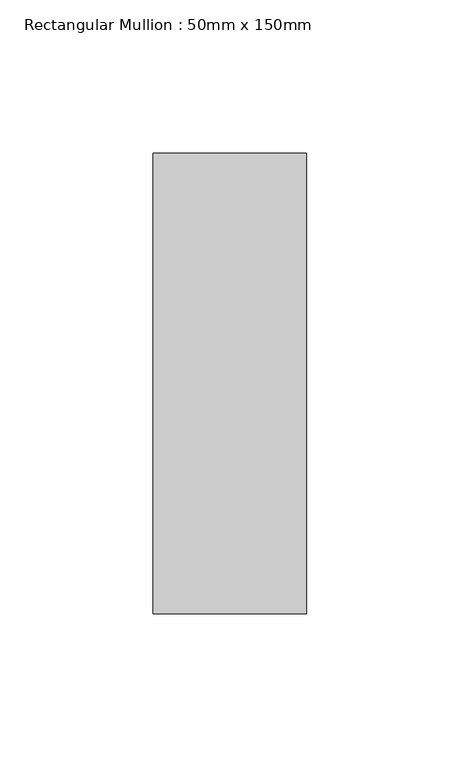
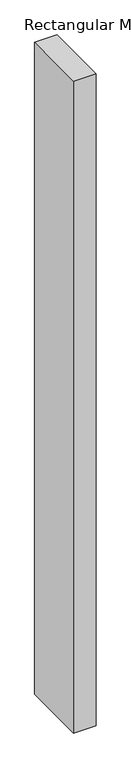
"""IFC4 building model written with IfcOpenShell, lengths in millimetres: member geometry, Rectangular Mullion : 50mm x 150mm."""

from ifc_helpers import new_model, si_unit, frame, origin, place, context, project, spatial, polyline, outline, extrude, source, transform, mapped, element, save


def rectangular_mullion_50mm_x_150mm_95afd124(model_context):
    return source(origin(), model_context, "Body", "SweptSolid", [
        extrude(outline(polyline([(0.0, 75.0), (0.0, -75.0), (-50.0, -75.0), (-50.0, 75.0), (0.0, 75.0)])), frame((0.0, 0.0, -1534.1021437), z_axis=(0.0, 0.0, 1.0), x_axis=(1.0, 0.0, 0.0)), (0.0, 0.0, 1.0), 1534.1021437),
    ])


if __name__ == "__main__":
    model = new_model("IFC4")
    model_context = context("Model", 3, world=origin())
    ifc_project = project(units=[si_unit("LENGTHUNIT", "METRE", prefix="MILLI")], contexts=[model_context])
    site = spatial("IfcSite", under=ifc_project)
    building = spatial("IfcBuilding", under=site)
    placement = place(None, origin())
    rectangular_mullion_50mm_x_150mm_shape = rectangular_mullion_50mm_x_150mm_95afd124(model_context)
    element("IfcMember", 1, ObjectType="Rectangular Mullion : 50mm x 150mm", at=placement, inside=building, context=model_context, shape_type="MappedRepresentation", body=[
        mapped(rectangular_mullion_50mm_x_150mm_shape, transform((0.0, 0.0, 0.0), x_axis=(1.0, 0.0, 0.0), y_axis=(0.0, 1.0, 0.0), z_axis=(0.0, 0.0, 1.0))),
    ])
    save(model, "model.ifc")

# Revit data of these elements
# Type "Rectangular Mullion : 50mm x 150mm"
#   built-in parameter 1007304 = 0.492126 (stored number, unit not read)
#   built-in parameter 1007301 = 0.082021 (stored number, unit not read)
#   built-in parameter 1007300 = 0.082021 (stored number, unit not read)
# Element 1 (IfcMember, "Rectangular Mullion : 50mm x 150mm")
#   Materials on its faces: "Aluminum"
# Materials
#   "Aluminum": class "Metal", colour RGB 247 247 247, transparency 0, Description = "Aluminum 6061", Cost = 0
